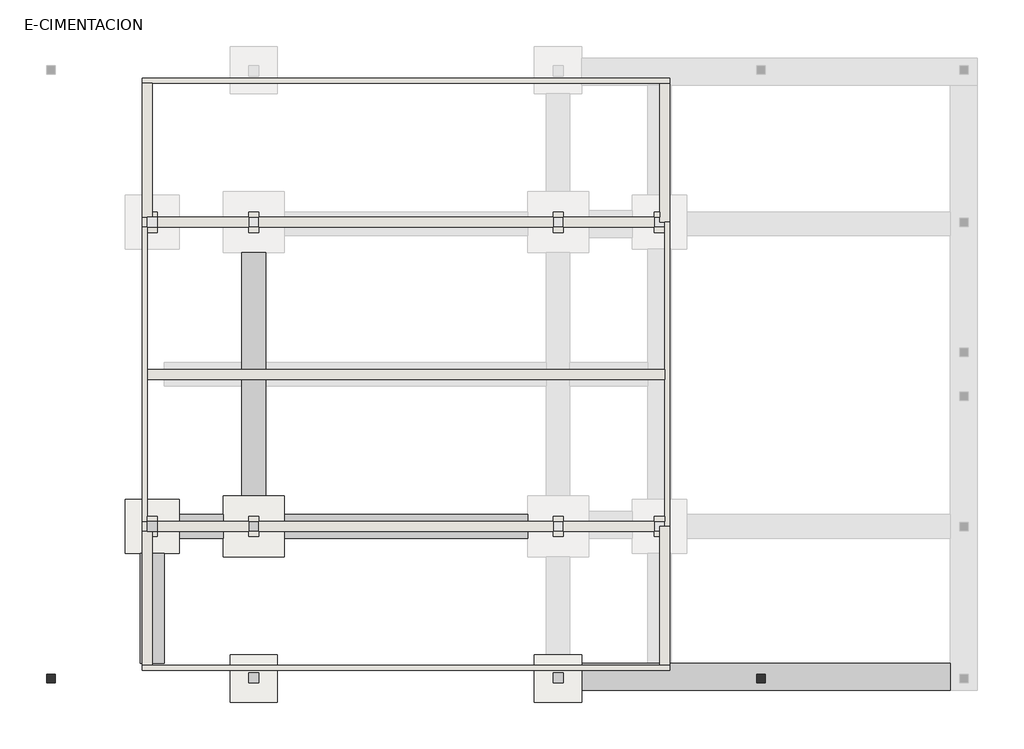
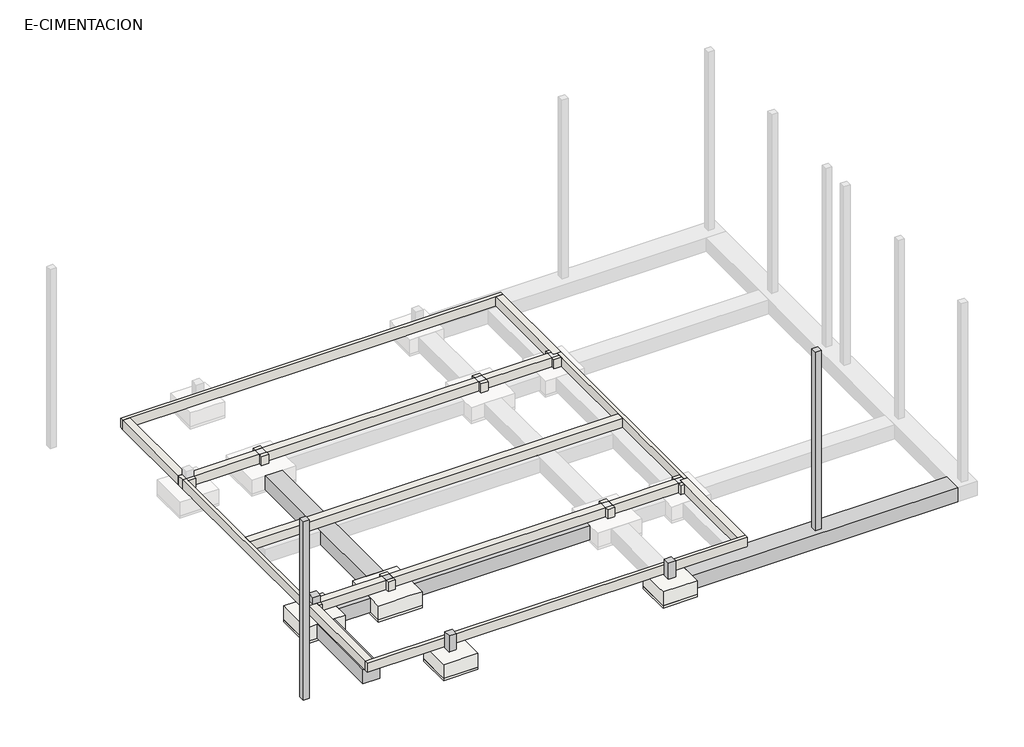
# One storey, part 1 of 2: 31 walls, 6 columns, 5 beams, 4 slabs.
"""IFC4 building model written with IfcOpenShell, lengths in millimetres."""

from ifc_helpers import new_model, si_unit, frame, origin, place, context, project, spatial, polyline, outline, extrude, faceted_brep, element, save

model = new_model("IFC4")

# Units and contexts
model_context = context("Model", 3, world=origin())
ifc_project = project(units=[si_unit("LENGTHUNIT", "METRE", prefix="MILLI")], contexts=[model_context])

# Site, building, storey
site = spatial("IfcSite", under=ifc_project)
building = spatial("IfcBuilding", under=site)
storey = spatial("IfcBuildingStorey", under=building, Name="E-CIMENTACION", Elevation=-900.0)

# Beams
placement = place(None, origin())
element("IfcBeam", 1, ObjectType="E-VIGA-Hormigon : E-VIGA-Hormigon", at=placement, inside=storey, context=model_context, shape_type="Brep", body=[
    faceted_brep([(-400.0, -17550.0, -900.0), (-400.0, -17550.0, -1500.0), (-8650.0, -17550.0, -1500.0), (-9350.0, -17550.0, -1500.0), (-11300.0, -17550.0, -1500.0), (-11300.0, -17550.0, -900.0), (-9350.0, -17550.0, -900.0), (-8650.0, -17550.0, -900.0), (-400.0, -18350.0, -1500.0), (-11300.0, -18350.0, -1500.0), (-400.0, -18350.0, -900.0), (-11300.0, -18350.0, -900.0)], [[[0, 1, 2, 3, 4, 5, 6, 7]], [[1, 8, 9, 4, 3, 2]], [[8, 10, 11, 9]], [[10, 0, 7, 6, 5, 11]], [[1, 0, 10, 8]], [[5, 4, 9, 11]]]),
])
element("IfcBeam", 2, ObjectType="E-VIGA-Hormigon : E-VIGA-Hormigon", at=placement, inside=storey, context=model_context, shape_type="SweptSolid", body=[
    extrude(outline(polyline([(-20100.0, -13850.0), (-20100.0, -13150.0), (-12900.0, -13150.0), (-12900.0, -13850.0), (-20100.0, -13850.0)])), frame((0.0, 0.0, -1500.0), z_axis=(0.0, 0.0, 1.0), x_axis=(1.0, 0.0, 0.0)), (0.0, 0.0, 1.0), 600.0),
])
element("IfcBeam", 3, ObjectType="E-VIGA-Hormigon : E-VIGA-Hormigon", at=placement, inside=storey, context=model_context, shape_type="SweptSolid", body=[
    extrude(outline(polyline([(-21900.0, -13150.0), (-21900.0, -13850.0), (-23200.0, -13850.0), (-23200.0, -13150.0), (-21900.0, -13150.0)])), frame((0.0, 0.0, -1500.0), z_axis=(0.0, 0.0, 1.0), x_axis=(1.0, 0.0, 0.0)), (0.0, 0.0, 1.0), 600.0),
])
element("IfcBeam", 4, ObjectType="E-VIGA-Hormigon : E-VIGA-Hormigon", at=placement, inside=storey, context=model_context, shape_type="Brep", body=[
    faceted_brep([(-20650.0, -5400.0, -1500.0), (-20650.0, -5400.0, -900.0), (-20650.0, -8650.0, -900.0), (-20650.0, -9350.0, -900.0), (-20650.0, -12600.0, -900.0), (-20650.0, -12600.0, -1500.0), (-20650.0, -9350.0, -1500.0), (-20650.0, -8650.0, -1500.0), (-21350.0, -5400.0, -1500.0), (-21350.0, -12600.0, -1500.0), (-21350.0, -9350.0, -1500.0), (-21350.0, -8650.0, -1500.0), (-21350.0, -5400.0, -900.0), (-21350.0, -12600.0, -900.0), (-21350.0, -9350.0, -900.0), (-21350.0, -8650.0, -900.0)], [[[0, 1, 2, 3, 4, 5, 6, 7]], [[8, 0, 7, 6, 5, 9, 10, 11]], [[12, 8, 11, 10, 9, 13, 14, 15]], [[1, 12, 15, 14, 13, 4, 3, 2]], [[1, 0, 8, 12]], [[5, 4, 13, 9]]]),
])
element("IfcBeam", 5, ObjectType="E-VIGA-Hormigon : E-VIGA-Hormigon", at=placement, inside=storey, context=model_context, shape_type="SweptSolid", body=[
    extrude(outline(polyline([(-24350.0, -14300.0), (-23650.0, -14300.0), (-23650.0, -17550.0), (-24350.0, -17550.0), (-24350.0, -14300.0)])), frame((0.0, 0.0, -1500.0), z_axis=(0.0, 0.0, 1.0), x_axis=(1.0, 0.0, 0.0)), (0.0, 0.0, 1.0), 600.0),
])

# Columns
element("IfcColumn", 6, ObjectType="Hormigón-Cuadrado-Pilar : PILAR 25X25", at=placement, inside=storey, context=model_context, shape_type="SweptSolid", body=[
    extrude(outline(polyline([(-26875.0, -17875.0), (-26875.0, -18125.0), (-27125.0, -18125.0), (-27125.0, -17875.0), (-26875.0, -17875.0)])), frame((0.0, 0.0, -900.0), z_axis=(0.0, 0.0, 1.0), x_axis=(1.0, 0.0, 0.0)), (0.0, 0.0, 1.0), 7750.0),
])
element("IfcColumn", 7, ObjectType="Hormigón-Cuadrado-Pilar : PILAR 25X25", at=placement, inside=storey, context=model_context, shape_type="SweptSolid", body=[
    extrude(outline(polyline([(-5875.0, -17875.0), (-5875.0, -18125.0), (-6125.0, -18125.0), (-6125.0, -17875.0), (-5875.0, -17875.0)])), frame((0.0, 0.0, -900.0), z_axis=(0.0, 0.0, 1.0), x_axis=(1.0, 0.0, 0.0)), (0.0, 0.0, 1.0), 7750.0),
])
element("IfcColumn", 8, ObjectType="Hormigón-Cuadrado-Pilar : PILAR 30X30", at=placement, inside=storey, context=model_context, shape_type="SweptSolid", body=[
    extrude(outline(polyline([(-20850.0, -18125.0), (-21150.0, -18125.0), (-21150.0, -17825.0), (-20850.0, -17825.0), (-20850.0, -18125.0)])), frame((0.0, 0.0, -900.0), z_axis=(0.0, 0.0, 1.0), x_axis=(1.0, 0.0, 0.0)), (0.0, 0.0, 1.0), 700.0),
])
element("IfcColumn", 9, ObjectType="Hormigón-Cuadrado-Pilar : PILAR 30X30", at=placement, inside=storey, context=model_context, shape_type="SweptSolid", body=[
    extrude(outline(polyline([(-11850.0, -18125.0), (-12150.0, -18125.0), (-12150.0, -17825.0), (-11850.0, -17825.0), (-11850.0, -18125.0)])), frame((0.0, 0.0, -900.0), z_axis=(0.0, 0.0, 1.0), x_axis=(1.0, 0.0, 0.0)), (0.0, 0.0, 1.0), 700.0),
])
element("IfcColumn", 10, ObjectType="Hormigón-Cuadrado-Pilar : PILAR 30X30", at=placement, inside=storey, context=model_context, shape_type="SweptSolid", body=[
    extrude(outline(polyline([(-20850.0, -13350.0), (-20850.0, -13650.0), (-21150.0, -13650.0), (-21150.0, -13350.0), (-20850.0, -13350.0)])), frame((0.0, 0.0, -900.0), z_axis=(0.0, 0.0, 1.0), x_axis=(1.0, 0.0, 0.0)), (0.0, 0.0, 1.0), 400.0),
])
element("IfcColumn", 11, ObjectType="Hormigón-Cuadrado-Pilar : PILAR 30X30", at=placement, inside=storey, context=model_context, shape_type="SweptSolid", body=[
    extrude(outline(polyline([(-23850.0, -13350.0), (-23850.0, -13650.0), (-24150.0, -13650.0), (-24150.0, -13350.0), (-23850.0, -13350.0)])), frame((0.0, 0.0, -500.0), z_axis=(0.0, 0.0, 1.0), x_axis=(1.0, 0.0, 0.0)), (0.0, 0.0, 1.0), 300.0),
])

# Slabs
element("IfcSlab", 12, ObjectType="E-ZAPATA : E-ZAPATA", at=placement, inside=storey, context=model_context, shape_type="SolidModel", body=[
    faceted_brep([(-21700.0, -18700.0, -900.0), (-20300.0, -18700.0, -900.0), (-20300.0, -18350.0, -900.0), (-20300.0, -17550.0, -900.0), (-20300.0, -17300.0, -900.0), (-20650.0, -17300.0, -900.0), (-21350.0, -17300.0, -900.0), (-21700.0, -17300.0, -900.0), (-21700.0, -17550.0, -900.0), (-21700.0, -18350.0, -900.0), (-21700.0, -18700.0, -1500.0), (-21700.0, -18350.0, -1500.0), (-21700.0, -17550.0, -1500.0), (-21700.0, -17300.0, -1500.0), (-21350.0, -17300.0, -1500.0), (-20650.0, -17300.0, -1500.0), (-20300.0, -17300.0, -1500.0), (-20300.0, -17550.0, -1500.0), (-20300.0, -18350.0, -1500.0), (-20300.0, -18700.0, -1500.0)], [[[0, 1, 2, 3, 4, 5, 6, 7, 8, 9]], [[10, 11, 12, 13, 14, 15, 16, 17, 18, 19]], [[0, 10, 19, 1]], [[1, 19, 18, 17, 16, 4, 3, 2]], [[4, 16, 15, 14, 13, 7, 6, 5]], [[7, 13, 12, 11, 10, 0, 9, 8]]]),
    extrude(outline(polyline([(-20300.0, -18700.0), (-21700.0, -18700.0), (-21700.0, -17300.0), (-20300.0, -17300.0), (-20300.0, -18700.0)])), frame((0.0, 0.0, -1600.0), z_axis=(0.0, 0.0, 1.0), x_axis=(1.0, 0.0, 0.0)), (0.0, 0.0, 1.0), 100.0),
])
element("IfcSlab", 13, ObjectType="E-ZAPATA : E-ZAPATA", at=placement, inside=storey, context=model_context, shape_type="SolidModel", body=[
    faceted_brep([(-12700.0, -18700.0, -900.0), (-11300.0, -18700.0, -900.0), (-11300.0, -18350.0, -900.0), (-11300.0, -17550.0, -900.0), (-11300.0, -17300.0, -900.0), (-11650.0, -17300.0, -900.0), (-12350.0, -17300.0, -900.0), (-12700.0, -17300.0, -900.0), (-12700.0, -17550.0, -900.0), (-12700.0, -18350.0, -900.0), (-12700.0, -18700.0, -1500.0), (-12700.0, -18350.0, -1500.0), (-12700.0, -17550.0, -1500.0), (-12700.0, -17300.0, -1500.0), (-12350.0, -17300.0, -1500.0), (-11650.0, -17300.0, -1500.0), (-11300.0, -17300.0, -1500.0), (-11300.0, -17550.0, -1500.0), (-11300.0, -18350.0, -1500.0), (-11300.0, -18700.0, -1500.0)], [[[0, 1, 2, 3, 4, 5, 6, 7, 8, 9]], [[10, 11, 12, 13, 14, 15, 16, 17, 18, 19]], [[0, 10, 19, 1]], [[1, 19, 18, 17, 16, 4, 3, 2]], [[4, 16, 15, 14, 13, 7, 6, 5]], [[7, 13, 12, 11, 10, 0, 9, 8]]]),
    extrude(outline(polyline([(-11300.0, -18700.0), (-12700.0, -18700.0), (-12700.0, -17300.0), (-11300.0, -17300.0), (-11300.0, -18700.0)])), frame((0.0, 0.0, -1600.0), z_axis=(0.0, 0.0, 1.0), x_axis=(1.0, 0.0, 0.0)), (0.0, 0.0, 1.0), 100.0),
])
element("IfcSlab", 14, ObjectType="E-ZAPATA : E-ZAPATA", at=placement, inside=storey, context=model_context, shape_type="SolidModel", body=[
    faceted_brep([(-21900.0, -14400.0, -900.0), (-21350.0, -14400.0, -900.0), (-20650.0, -14400.0, -900.0), (-20100.0, -14400.0, -900.0), (-20100.0, -13850.0, -900.0), (-20100.0, -13150.0, -900.0), (-20100.0, -12600.0, -900.0), (-20650.0, -12600.0, -900.0), (-21350.0, -12600.0, -900.0), (-21900.0, -12600.0, -900.0), (-21900.0, -13150.0, -900.0), (-21900.0, -13850.0, -900.0), (-21900.0, -14400.0, -1500.0), (-21900.0, -13850.0, -1500.0), (-21900.0, -13150.0, -1500.0), (-21900.0, -12600.0, -1500.0), (-21350.0, -12600.0, -1500.0), (-20650.0, -12600.0, -1500.0), (-20100.0, -12600.0, -1500.0), (-20100.0, -13150.0, -1500.0), (-20100.0, -13850.0, -1500.0), (-20100.0, -14400.0, -1500.0), (-20650.0, -14400.0, -1500.0), (-21350.0, -14400.0, -1500.0)], [[[0, 1, 2, 3, 4, 5, 6, 7, 8, 9, 10, 11]], [[12, 13, 14, 15, 16, 17, 18, 19, 20, 21, 22, 23]], [[0, 12, 23, 22, 21, 3, 2, 1]], [[3, 21, 20, 19, 18, 6, 5, 4]], [[6, 18, 17, 16, 15, 9, 8, 7]], [[9, 15, 14, 13, 12, 0, 11, 10]]]),
    extrude(outline(polyline([(-20100.0, -14400.0), (-21900.0, -14400.0), (-21900.0, -12600.0), (-20100.0, -12600.0), (-20100.0, -14400.0)])), frame((0.0, 0.0, -1600.0), z_axis=(0.0, 0.0, 1.0), x_axis=(1.0, 0.0, 0.0)), (0.0, 0.0, 1.0), 100.0),
])
element("IfcSlab", 15, ObjectType="E-ZAPATA : E-ZAPATA", at=placement, inside=storey, context=model_context, shape_type="SolidModel", body=[
    faceted_brep([(-24800.0, -14300.0, -900.0), (-24350.0, -14300.0, -900.0), (-23650.0, -14300.0, -900.0), (-23200.0, -14300.0, -900.0), (-23200.0, -13850.0, -900.0), (-23200.0, -13150.0, -900.0), (-23200.0, -12700.0, -900.0), (-23650.0, -12700.0, -900.0), (-24350.0, -12700.0, -900.0), (-24800.0, -12700.0, -900.0), (-24800.0, -14300.0, -1500.0), (-24800.0, -12700.0, -1500.0), (-24350.0, -12700.0, -1500.0), (-23650.0, -12700.0, -1500.0), (-23200.0, -12700.0, -1500.0), (-23200.0, -13150.0, -1500.0), (-23200.0, -13850.0, -1500.0), (-23200.0, -14300.0, -1500.0), (-23650.0, -14300.0, -1500.0), (-24350.0, -14300.0, -1500.0)], [[[0, 1, 2, 3, 4, 5, 6, 7, 8, 9]], [[10, 11, 12, 13, 14, 15, 16, 17, 18, 19]], [[0, 10, 19, 18, 17, 3, 2, 1]], [[3, 17, 16, 15, 14, 6, 5, 4]], [[6, 14, 13, 12, 11, 9, 8, 7]], [[9, 11, 10, 0]]]),
    extrude(outline(polyline([(-23200.0, -14300.0), (-24800.0, -14300.0), (-24800.0, -12700.0), (-23200.0, -12700.0), (-23200.0, -14300.0)])), frame((0.0, 0.0, -1600.0), z_axis=(0.0, 0.0, 1.0), x_axis=(1.0, 0.0, 0.0)), (0.0, 0.0, 1.0), 100.0),
])

# Walls
element("IfcWall", 16, ObjectType="MURETE FORJ SAN 1 PIE_PABLO", at=placement, inside=storey, context=model_context, shape_type="SweptSolid", body=[
    extrude(outline(polyline([(-12150.0, -13650.0), (-20850.0, -13650.0), (-20850.0, -13350.0), (-12150.0, -13350.0), (-12150.0, -13650.0)])), frame((0.0, 0.0, -900.0), z_axis=(0.0, 0.0, 1.0), x_axis=(1.0, 0.0, 0.0)), (0.0, 0.0, 1.0), 400.0),
])
element("IfcWall", 17, ObjectType="MURETE FORJ SAN 1 PIE_PABLO", at=placement, inside=storey, context=model_context, shape_type="Brep", body=[
    faceted_brep([(-24300.0, -13650.0, -900.0), (-24000.0, -13650.0, -900.0), (-21150.0, -13650.0, -900.0), (-21150.0, -13650.0, -500.0), (-23850.0, -13650.0, -500.0), (-24000.0, -13650.0, -500.0), (-24150.0, -13650.0, -500.0), (-24300.0, -13650.0, -500.0), (-24300.0, -13350.0, -900.0), (-24300.0, -13350.0, -500.0), (-24150.0, -13350.0, -500.0), (-23850.0, -13350.0, -500.0), (-21150.0, -13350.0, -500.0), (-21150.0, -13350.0, -900.0), (-24150.0, -13350.0, -900.0)], [[[0, 1, 2, 3, 4, 5, 6, 7]], [[8, 9, 10, 11, 12, 13, 14]], [[2, 1, 0, 8, 14, 13]], [[3, 2, 13, 12]], [[7, 6, 5, 4, 3, 12, 11, 10, 9]], [[0, 7, 9, 8]]]),
])
element("IfcWall", 18, ObjectType="MURETE FORJ SAN 1 PIE_PABLO", at=placement, inside=storey, context=model_context, shape_type="SweptSolid", body=[
    extrude(outline(polyline([(-9150.0, -13650.0), (-11850.0, -13650.0), (-11850.0, -13350.0), (-9150.0, -13350.0), (-9150.0, -13650.0)])), frame((0.0, 0.0, -900.0), z_axis=(0.0, 0.0, 1.0), x_axis=(1.0, 0.0, 0.0)), (0.0, 0.0, 1.0), 400.0),
])
element("IfcWall", 19, ObjectType="MURETE FORJ SAN 1 PIE_PABLO", at=placement, inside=storey, context=model_context, shape_type="SweptSolid", body=[
    extrude(outline(polyline([(-8850.0, -9150.0), (-24150.0, -9150.0), (-24150.0, -8850.0), (-8850.0, -8850.0), (-8850.0, -9150.0)])), frame((0.0, 0.0, -900.0), z_axis=(0.0, 0.0, 1.0), x_axis=(1.0, 0.0, 0.0)), (0.0, 0.0, 1.0), 400.0),
])
element("IfcWall", 20, ObjectType="MURETE FORJ SAN 1 PIE_PABLO", at=placement, inside=storey, context=model_context, shape_type="Brep", body=[
    faceted_brep([(-24300.0, -4650.0, -900.0), (-24150.0, -4650.0, -900.0), (-21150.0, -4650.0, -900.0), (-21150.0, -4650.0, -500.0), (-23850.0, -4650.0, -500.0), (-24150.0, -4650.0, -500.0), (-24300.0, -4650.0, -500.0), (-24300.0, -4350.0, -900.0), (-24300.0, -4350.0, -500.0), (-24150.0, -4350.0, -500.0), (-24000.0, -4350.0, -500.0), (-23850.0, -4350.0, -500.0), (-21150.0, -4350.0, -500.0), (-21150.0, -4350.0, -900.0), (-24000.0, -4350.0, -900.0)], [[[0, 1, 2, 3, 4, 5, 6]], [[7, 8, 9, 10, 11, 12, 13, 14]], [[2, 1, 0, 7, 14, 13]], [[3, 2, 13, 12]], [[6, 5, 4, 3, 12, 11, 10, 9, 8]], [[0, 6, 8, 7]]]),
])
element("IfcWall", 21, ObjectType="MURETE FORJ SAN 1 PIE_PABLO", at=placement, inside=storey, context=model_context, shape_type="SweptSolid", body=[
    extrude(outline(polyline([(-12150.0, -4650.0), (-20850.0, -4650.0), (-20850.0, -4350.0), (-12150.0, -4350.0), (-12150.0, -4650.0)])), frame((0.0, 0.0, -900.0), z_axis=(0.0, 0.0, 1.0), x_axis=(1.0, 0.0, 0.0)), (0.0, 0.0, 1.0), 400.0),
])
element("IfcWall", 22, ObjectType="MURETE FORJ SAN 1 PIE_PABLO", at=placement, inside=storey, context=model_context, shape_type="SweptSolid", body=[
    extrude(outline(polyline([(-9150.0, -4650.0), (-11850.0, -4650.0), (-11850.0, -4350.0), (-9150.0, -4350.0), (-9150.0, -4650.0)])), frame((0.0, 0.0, -900.0), z_axis=(0.0, 0.0, 1.0), x_axis=(1.0, 0.0, 0.0)), (0.0, 0.0, 1.0), 400.0),
])
element("IfcWall", 23, ObjectType="MURETE FORJ SAN 1/2 PIE_PABLO", at=placement, inside=storey, context=model_context, shape_type="Brep", body=[
    faceted_brep([(-24300.0, -387.5, -900.0), (-24000.0, -387.5, -900.0), (-9000.0, -387.5, -900.0), (-8700.0, -387.5, -900.0), (-8700.0, -387.5, -500.0), (-9000.0, -387.5, -500.0), (-24000.0, -387.5, -500.0), (-24300.0, -387.5, -500.0), (-24300.0, -237.5, -900.0), (-24300.0, -237.5, -500.0), (-8700.0, -237.5, -500.0), (-8700.0, -237.5, -900.0)], [[[0, 1, 2, 3, 4, 5, 6, 7]], [[8, 9, 10, 11]], [[3, 2, 1, 0, 8, 11]], [[7, 6, 5, 4, 10, 9]], [[0, 7, 9, 8]], [[4, 3, 11, 10]]]),
])
element("IfcWall", 24, ObjectType="MURETE FORJ SAN 1 PIE_PABLO", at=placement, inside=storey, context=model_context, shape_type="Brep", body=[
    faceted_brep([(-24000.0, -4350.0, -900.0), (-24000.0, -4200.0, -900.0), (-24000.0, -387.5, -900.0), (-24000.0, -387.5, -500.0), (-24000.0, -4200.0, -500.0), (-24000.0, -4350.0, -500.0), (-24300.0, -4350.0, -900.0), (-24300.0, -4350.0, -500.0), (-24300.0, -387.5, -500.0), (-24300.0, -387.5, -900.0)], [[[0, 1, 2, 3, 4, 5]], [[6, 7, 8, 9]], [[2, 1, 0, 6, 9]], [[5, 4, 3, 8, 7]], [[3, 2, 9, 8]], [[0, 5, 7, 6]]]),
])
element("IfcWall", 25, ObjectType="MURETE FORJ SAN 1/2 PIE_PABLO", at=placement, inside=storey, context=model_context, shape_type="Brep", body=[
    faceted_brep([(-24300.0, -17762.5, -900.0), (-8700.0, -17762.5, -900.0), (-8700.0, -17762.5, -500.0), (-24300.0, -17762.5, -500.0), (-24300.0, -17612.5, -900.0), (-24300.0, -17612.5, -500.0), (-24000.0, -17612.5, -500.0), (-9000.0, -17612.5, -500.0), (-8700.0, -17612.5, -500.0), (-8700.0, -17612.5, -900.0), (-9000.0, -17612.5, -900.0), (-24000.0, -17612.5, -900.0)], [[[0, 1, 2, 3]], [[4, 5, 6, 7, 8, 9, 10, 11]], [[1, 0, 4, 11, 10, 9]], [[3, 2, 8, 7, 6, 5]], [[0, 3, 5, 4]], [[2, 1, 9, 8]]]),
])
element("IfcWall", 26, ObjectType="MURETE FORJ SAN 1 PIE_PABLO", at=placement, inside=storey, context=model_context, shape_type="Brep", body=[
    faceted_brep([(-24000.0, -17612.5, -900.0), (-24000.0, -13800.0, -900.0), (-24000.0, -13650.0, -900.0), (-24000.0, -13650.0, -500.0), (-24000.0, -13800.0, -500.0), (-24000.0, -17612.5, -500.0), (-24300.0, -17612.5, -900.0), (-24300.0, -17612.5, -500.0), (-24300.0, -13650.0, -500.0), (-24300.0, -13650.0, -900.0)], [[[0, 1, 2, 3, 4, 5]], [[6, 7, 8, 9]], [[2, 1, 0, 6, 9]], [[5, 4, 3, 8, 7]], [[3, 2, 9, 8]], [[0, 5, 7, 6]]]),
])
element("IfcWall", 27, ObjectType="MURETE FORJ SAN 1/2 PIE_PABLO", at=placement, inside=storey, context=model_context, shape_type="Brep", body=[
    faceted_brep([(-24150.0, -13350.0, -900.0), (-24150.0, -13200.0, -900.0), (-24150.0, -9150.0, -900.0), (-24150.0, -8850.0, -900.0), (-24150.0, -4800.0, -900.0), (-24150.0, -4650.0, -900.0), (-24150.0, -4650.0, -500.0), (-24150.0, -4800.0, -500.0), (-24150.0, -8850.0, -500.0), (-24150.0, -9150.0, -500.0), (-24150.0, -13200.0, -500.0), (-24150.0, -13350.0, -500.0), (-24300.0, -13350.0, -900.0), (-24300.0, -13350.0, -500.0), (-24300.0, -4650.0, -500.0), (-24300.0, -4650.0, -900.0)], [[[0, 1, 2, 3, 4, 5, 6, 7, 8, 9, 10, 11]], [[12, 13, 14, 15]], [[5, 4, 3, 2, 1, 0, 12, 15]], [[11, 10, 9, 8, 7, 6, 14, 13]], [[0, 11, 13, 12]], [[6, 5, 15, 14]]]),
])
element("IfcWall", 28, ObjectType="MURETE FORJ SAN 1 PIE_PABLO", at=placement, inside=storey, context=model_context, shape_type="Brep", body=[
    faceted_brep([(-8700.0, -4500.0, -900.0), (-8700.0, -387.5, -900.0), (-8700.0, -387.5, -500.0), (-8700.0, -4500.0, -500.0), (-9000.0, -4500.0, -900.0), (-9000.0, -4500.0, -500.0), (-9000.0, -4350.0, -500.0), (-9000.0, -4200.0, -500.0), (-9000.0, -387.5, -500.0), (-9000.0, -387.5, -900.0), (-9000.0, -4200.0, -900.0), (-9000.0, -4350.0, -900.0), (-8850.0, -4500.0, -900.0), (-8850.0, -4500.0, -500.0)], [[[0, 1, 2, 3]], [[4, 5, 6, 7, 8, 9, 10, 11]], [[1, 0, 12, 4, 11, 10, 9]], [[3, 2, 8, 7, 6, 5, 13]], [[0, 3, 13, 5, 4, 12]], [[2, 1, 9, 8]]]),
])
element("IfcWall", 29, ObjectType="MURETE FORJ SAN 1 PIE_PABLO", at=placement, inside=storey, context=model_context, shape_type="Brep", body=[
    faceted_brep([(-8700.0, -17612.5, -900.0), (-8700.0, -13500.0, -900.0), (-8700.0, -13500.0, -500.0), (-8700.0, -17612.5, -500.0), (-9000.0, -17612.5, -900.0), (-9000.0, -17612.5, -500.0), (-9000.0, -13800.0, -500.0), (-9000.0, -13650.0, -500.0), (-9000.0, -13500.0, -500.0), (-9000.0, -13500.0, -900.0), (-9000.0, -13650.0, -900.0), (-9000.0, -13800.0, -900.0), (-8850.0, -13500.0, -900.0), (-8850.0, -13500.0, -500.0)], [[[0, 1, 2, 3]], [[4, 5, 6, 7, 8, 9, 10, 11]], [[1, 0, 4, 11, 10, 9, 12]], [[2, 1, 12, 9, 8, 13]], [[3, 2, 13, 8, 7, 6, 5]], [[0, 3, 5, 4]]]),
])
element("IfcWall", 30, ObjectType="MURETE FORJ SAN 1/2 PIE_PABLO", at=placement, inside=storey, context=model_context, shape_type="Brep", body=[
    faceted_brep([(-8700.0, -13500.0, -900.0), (-8700.0, -4500.0, -900.0), (-8700.0, -4500.0, -500.0), (-8700.0, -13500.0, -500.0), (-8850.0, -13500.0, -900.0), (-8850.0, -13500.0, -500.0), (-8850.0, -13350.0, -500.0), (-8850.0, -13200.0, -500.0), (-8850.0, -9150.0, -500.0), (-8850.0, -8850.0, -500.0), (-8850.0, -4800.0, -500.0), (-8850.0, -4650.0, -500.0), (-8850.0, -4500.0, -500.0), (-8850.0, -4500.0, -900.0), (-8850.0, -4650.0, -900.0), (-8850.0, -4800.0, -900.0), (-8850.0, -8850.0, -900.0), (-8850.0, -9150.0, -900.0), (-8850.0, -13200.0, -900.0), (-8850.0, -13350.0, -900.0)], [[[0, 1, 2, 3]], [[4, 5, 6, 7, 8, 9, 10, 11, 12, 13, 14, 15, 16, 17, 18, 19]], [[1, 0, 4, 19, 18, 17, 16, 15, 14, 13]], [[2, 1, 13, 12]], [[3, 2, 12, 11, 10, 9, 8, 7, 6, 5]], [[0, 3, 5, 4]]]),
])
element("IfcWall", 31, ObjectType="MURETE FORJ SAN 1/2 PIE_PABLO", at=placement, inside=storey, context=model_context, shape_type="SweptSolid", body=[
    extrude(outline(polyline([(-23850.0, -4800.0), (-24150.0, -4800.0), (-24150.0, -4650.0), (-23850.0, -4650.0), (-23850.0, -4800.0)])), frame((0.0, 0.0, -900.0), z_axis=(0.0, 0.0, 1.0), x_axis=(1.0, 0.0, 0.0)), (0.0, 0.0, 1.0), 400.0),
])
element("IfcWall", 32, ObjectType="MURETE FORJ SAN 1/2 PIE_PABLO", at=placement, inside=storey, context=model_context, shape_type="SweptSolid", body=[
    extrude(outline(polyline([(-23850.0, -4350.0), (-24000.0, -4350.0), (-24000.0, -4200.0), (-23850.0, -4200.0), (-23850.0, -4350.0)])), frame((0.0, 0.0, -900.0), z_axis=(0.0, 0.0, 1.0), x_axis=(1.0, 0.0, 0.0)), (0.0, 0.0, 1.0), 400.0),
])
element("IfcWall", 33, ObjectType="MURETE FORJ SAN 1/2 PIE_PABLO", at=placement, inside=storey, context=model_context, shape_type="SweptSolid", body=[
    extrude(outline(polyline([(-20850.0, -4350.0), (-21150.0, -4350.0), (-21150.0, -4200.0), (-20850.0, -4200.0), (-20850.0, -4350.0)])), frame((0.0, 0.0, -900.0), z_axis=(0.0, 0.0, 1.0), x_axis=(1.0, 0.0, 0.0)), (0.0, 0.0, 1.0), 400.0),
])
element("IfcWall", 34, ObjectType="MURETE FORJ SAN 1/2 PIE_PABLO", at=placement, inside=storey, context=model_context, shape_type="SweptSolid", body=[
    extrude(outline(polyline([(-20850.0, -4800.0), (-21150.0, -4800.0), (-21150.0, -4650.0), (-20850.0, -4650.0), (-20850.0, -4800.0)])), frame((0.0, 0.0, -900.0), z_axis=(0.0, 0.0, 1.0), x_axis=(1.0, 0.0, 0.0)), (0.0, 0.0, 1.0), 400.0),
])
element("IfcWall", 35, ObjectType="MURETE FORJ SAN 1/2 PIE_PABLO", at=placement, inside=storey, context=model_context, shape_type="SweptSolid", body=[
    extrude(outline(polyline([(-9150.0, -4650.0), (-8850.0, -4650.0), (-8850.0, -4800.0), (-9150.0, -4800.0), (-9150.0, -4650.0)])), frame((0.0, 0.0, -900.0), z_axis=(0.0, 0.0, 1.0), x_axis=(1.0, 0.0, 0.0)), (0.0, 0.0, 1.0), 400.0),
])
element("IfcWall", 36, ObjectType="MURETE FORJ SAN 1/2 PIE_PABLO", at=placement, inside=storey, context=model_context, shape_type="SweptSolid", body=[
    extrude(outline(polyline([(-9150.0, -4200.0), (-9000.0, -4200.0), (-9000.0, -4350.0), (-9150.0, -4350.0), (-9150.0, -4200.0)])), frame((0.0, 0.0, -900.0), z_axis=(0.0, 0.0, 1.0), x_axis=(1.0, 0.0, 0.0)), (0.0, 0.0, 1.0), 400.0),
])
element("IfcWall", 37, ObjectType="MURETE FORJ SAN 1/2 PIE_PABLO", at=placement, inside=storey, context=model_context, shape_type="SweptSolid", body=[
    extrude(outline(polyline([(-12150.0, -4200.0), (-11850.0, -4200.0), (-11850.0, -4350.0), (-12150.0, -4350.0), (-12150.0, -4200.0)])), frame((0.0, 0.0, -900.0), z_axis=(0.0, 0.0, 1.0), x_axis=(1.0, 0.0, 0.0)), (0.0, 0.0, 1.0), 400.0),
])
element("IfcWall", 38, ObjectType="MURETE FORJ SAN 1/2 PIE_PABLO", at=placement, inside=storey, context=model_context, shape_type="SweptSolid", body=[
    extrude(outline(polyline([(-12150.0, -4650.0), (-11850.0, -4650.0), (-11850.0, -4800.0), (-12150.0, -4800.0), (-12150.0, -4650.0)])), frame((0.0, 0.0, -900.0), z_axis=(0.0, 0.0, 1.0), x_axis=(1.0, 0.0, 0.0)), (0.0, 0.0, 1.0), 400.0),
])
element("IfcWall", 39, ObjectType="MURETE FORJ SAN 1/2 PIE_PABLO", at=placement, inside=storey, context=model_context, shape_type="SweptSolid", body=[
    extrude(outline(polyline([(-23850.0, -13350.0), (-24150.0, -13350.0), (-24150.0, -13200.0), (-23850.0, -13200.0), (-23850.0, -13350.0)])), frame((0.0, 0.0, -900.0), z_axis=(0.0, 0.0, 1.0), x_axis=(1.0, 0.0, 0.0)), (0.0, 0.0, 1.0), 400.0),
])
element("IfcWall", 40, ObjectType="MURETE FORJ SAN 1/2 PIE_PABLO", at=placement, inside=storey, context=model_context, shape_type="SweptSolid", body=[
    extrude(outline(polyline([(-23850.0, -13800.0), (-24000.0, -13800.0), (-24000.0, -13650.0), (-23850.0, -13650.0), (-23850.0, -13800.0)])), frame((0.0, 0.0, -900.0), z_axis=(0.0, 0.0, 1.0), x_axis=(1.0, 0.0, 0.0)), (0.0, 0.0, 1.0), 400.0),
])
element("IfcWall", 41, ObjectType="MURETE FORJ SAN 1/2 PIE_PABLO", at=placement, inside=storey, context=model_context, shape_type="SweptSolid", body=[
    extrude(outline(polyline([(-20850.0, -13800.0), (-21150.0, -13800.0), (-21150.0, -13650.0), (-20850.0, -13650.0), (-20850.0, -13800.0)])), frame((0.0, 0.0, -900.0), z_axis=(0.0, 0.0, 1.0), x_axis=(1.0, 0.0, 0.0)), (0.0, 0.0, 1.0), 400.0),
])
element("IfcWall", 42, ObjectType="MURETE FORJ SAN 1/2 PIE_PABLO", at=placement, inside=storey, context=model_context, shape_type="SweptSolid", body=[
    extrude(outline(polyline([(-20850.0, -13350.0), (-21150.0, -13350.0), (-21150.0, -13200.0), (-20850.0, -13200.0), (-20850.0, -13350.0)])), frame((0.0, 0.0, -900.0), z_axis=(0.0, 0.0, 1.0), x_axis=(1.0, 0.0, 0.0)), (0.0, 0.0, 1.0), 400.0),
])
element("IfcWall", 43, ObjectType="MURETE FORJ SAN 1/2 PIE_PABLO", at=placement, inside=storey, context=model_context, shape_type="SweptSolid", body=[
    extrude(outline(polyline([(-9150.0, -13200.0), (-8850.0, -13200.0), (-8850.0, -13350.0), (-9150.0, -13350.0), (-9150.0, -13200.0)])), frame((0.0, 0.0, -900.0), z_axis=(0.0, 0.0, 1.0), x_axis=(1.0, 0.0, 0.0)), (0.0, 0.0, 1.0), 400.0),
])
element("IfcWall", 44, ObjectType="MURETE FORJ SAN 1/2 PIE_PABLO", at=placement, inside=storey, context=model_context, shape_type="SweptSolid", body=[
    extrude(outline(polyline([(-9150.0, -13650.0), (-9000.0, -13650.0), (-9000.0, -13800.0), (-9150.0, -13800.0), (-9150.0, -13650.0)])), frame((0.0, 0.0, -900.0), z_axis=(0.0, 0.0, 1.0), x_axis=(1.0, 0.0, 0.0)), (0.0, 0.0, 1.0), 400.0),
])
element("IfcWall", 45, ObjectType="MURETE FORJ SAN 1/2 PIE_PABLO", at=placement, inside=storey, context=model_context, shape_type="SweptSolid", body=[
    extrude(outline(polyline([(-12150.0, -13650.0), (-11850.0, -13650.0), (-11850.0, -13800.0), (-12150.0, -13800.0), (-12150.0, -13650.0)])), frame((0.0, 0.0, -900.0), z_axis=(0.0, 0.0, 1.0), x_axis=(1.0, 0.0, 0.0)), (0.0, 0.0, 1.0), 400.0),
])
element("IfcWall", 46, ObjectType="MURETE FORJ SAN 1/2 PIE_PABLO", at=placement, inside=storey, context=model_context, shape_type="SweptSolid", body=[
    extrude(outline(polyline([(-12150.0, -13200.0), (-11850.0, -13200.0), (-11850.0, -13350.0), (-12150.0, -13350.0), (-12150.0, -13200.0)])), frame((0.0, 0.0, -900.0), z_axis=(0.0, 0.0, 1.0), x_axis=(1.0, 0.0, 0.0)), (0.0, 0.0, 1.0), 400.0),
])

save(model, "model.ifc")

# Revit data of these elements
# Type "E-VIGA-Hormigon : E-VIGA-Hormigon"
#   Numeration [instance default] = ""
#   Length [instance default] = 3.000 m
#   AnchoViga [instance default] = 0.200 m
#   AltoViga [instance default] = 0.300 m
# Type "Hormigón-Cuadrado-Pilar : PILAR 25X25"
#   b = 0.250 m
#   Structural Material [instance default] = Hormigón - Hormigón moldeado in situ
# Type "Hormigón-Cuadrado-Pilar : PILAR 30X30"
#   b = 0.300 m
#   Structural Material [instance default] = Hormigón - Hormigón moldeado in situ
# Type "E-ZAPATA : E-ZAPATA"
#   y1 [instance default] = 0.500 m
#   x1 [instance default] = 0.500 m
#   GrosorHormigonLimpieza [instance default] = 0.100 m
#   Width [instance default] = 1.000 m
#   Length [instance default] = 1.000 m
#   Foundation Thickness [instance default] = 0.500 m
#   ColocacionEjeY [instance default] = no
#   ColocacionEjeX [instance default] = no
#   HormigonLimpieza = none
#   Structural Material = none
# Type "MURETE FORJ SAN 1 PIE_PABLO"
#   Layers, outside or top first: 0.300 m "Ladrillo, hueco" (function 1)
# Type "MURETE FORJ SAN 1/2 PIE_PABLO"
#   Layers, outside or top first: 0.150 m "Ladrillo, hueco" (function 1)
# Element 1 (IfcBeam, "E-VIGA-Hormigon : E-VIGA-Hormigon")
#   Comments = ""
#   Numeration = ""
#   AnchoViga = 0.800 m
#   AltoViga = 0.600 m
#   Phase Created = Nueva construcción
#   Materials on its faces: "Concrete, Cast-in-Place, Gray"
# Elements 2, 3, 4, 5 (IfcBeam, "E-VIGA-Hormigon : E-VIGA-Hormigon")
#   Comments = ""
#   Numeration = ""
#   AnchoViga = 0.700 m
#   AltoViga = 0.600 m
#   Phase Created = Nueva construcción
#   Materials on its faces: "Concrete, Cast-in-Place, Gray"
# Elements 6, 7 (IfcColumn, "Hormigón-Cuadrado-Pilar : PILAR 25X25")
#   Comments = ""
#   Structural Material = Hormigón - Hormigón moldeado in situ
#   Phase Created = Nueva construcción
#   Materials on its faces: "Hormigón - Hormigón moldeado in situ"
# Elements 8, 9, 10, 11 (IfcColumn, "Hormigón-Cuadrado-Pilar : PILAR 30X30")
#   Comments = ""
#   Structural Material = Hormigón - Hormigón moldeado in situ
#   Phase Created = Nueva construcción
#   Materials on its faces: "Hormigón - Hormigón moldeado in situ"
# Elements 12, 13 (IfcSlab, "E-ZAPATA : E-ZAPATA")
#   Comments = ""
#   y1 = 0.700 m
#   x1 = 0.700 m
#   Length = 1.400 m
#   GrosorHormigonLimpieza = 0.100 m
#   Foundation Thickness = 0.600 m
#   Width = 1.400 m
#   ColocacionEjeY = no
#   ColocacionEjeX = no
#   Phase Created = Nueva construcción
# Element 14 (IfcSlab, "E-ZAPATA : E-ZAPATA")
#   Comments = ""
#   y1 = 0.900 m
#   x1 = 0.900 m
#   Length = 1.800 m
#   GrosorHormigonLimpieza = 0.100 m
#   Foundation Thickness = 0.600 m
#   Width = 1.800 m
#   ColocacionEjeY = no
#   ColocacionEjeX = no
#   Phase Created = Nueva construcción
# Element 15 (IfcSlab, "E-ZAPATA : E-ZAPATA")
#   Comments = ""
#   y1 = 0.800 m
#   x1 = 0.800 m
#   Length = 1.600 m
#   GrosorHormigonLimpieza = 0.100 m
#   Foundation Thickness = 0.600 m
#   Width = 1.600 m
#   ColocacionEjeY = no
#   ColocacionEjeX = no
#   Phase Created = Nueva construcción
# Elements 16, 17, 18, 19, 20, 21, 22, 24, 26, 28, 29 (IfcWall, "MURETE FORJ SAN 1 PIE_PABLO")
#   Comments = ""
#   Top Offset = 0.000 m
#   Base Offset = 0.000 m
#   Unconnected Height = 0.400 m
#   wall height = 0.400 m
#   Phase Created = Nueva construcción
#   Base Constraint = E-CIMENTACION
#   Materials on its faces: "Ladrillo, hueco"
# Elements 23, 25, 27, 30, 31, 32, 33, 34, 35, 36, 37, 38, 39, 40, 41, 42, 43, 44, 45, 46 (IfcWall, "MURETE FORJ SAN 1/2 PIE_PABLO")
#   Comments = ""
#   Top Offset = 0.000 m
#   Base Offset = 0.000 m
#   Unconnected Height = 0.400 m
#   wall height = 0.400 m
#   Phase Created = Nueva construcción
#   Base Constraint = E-CIMENTACION
#   Materials on its faces: "Ladrillo, hueco"
# Materials
#   "Hormigón - Hormigón moldeado in situ": class "Hormigón", colour RGB 192 192 192, transparency 0, Cost = 0
#   "Ladrillo, hueco": class "Albañilería", colour RGB 120 120 120, transparency 0, Description = "Ladrillo hueco", Cost = 0
#   "Concrete, Cast-in-Place, Gray": class "Concrete", colour RGB 129 132 118, transparency 0, Description = "Cast-in-place concrete", Cost = 0
